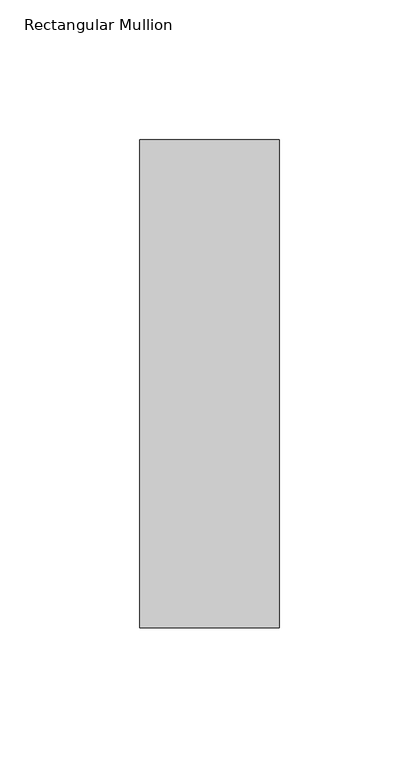
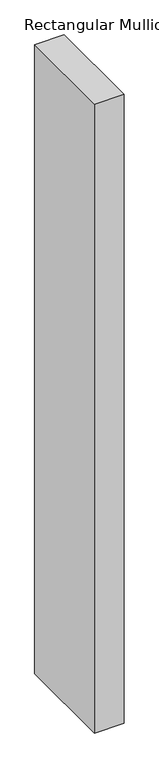
"""IFC4 building model written with IfcOpenShell, lengths in millimetres: member geometry, Rectangular Mullion : WWm-50x175-50mmOffset."""

from ifc_helpers import new_model, si_unit, frame, origin, place, context, project, spatial, polyline, outline, extrude, source, transform, mapped, element, save


def rectangular_mullion_8e94abb8(model_context):
    return source(origin(), model_context, "Body", "SweptSolid", [
        extrude(outline(polyline([(0.0, 87.5), (0.0, -87.5), (-50.0, -87.5), (-50.0, 87.5), (0.0, 87.5)])), frame((0.0, 0.0, -1125.0), z_axis=(0.0, 0.0, 1.0), x_axis=(1.0, 0.0, 0.0)), (0.0, 0.0, 1.0), 1125.0),
    ])


if __name__ == "__main__":
    model = new_model("IFC4")
    model_context = context("Model", 3, world=origin())
    ifc_project = project(units=[si_unit("LENGTHUNIT", "METRE", prefix="MILLI")], contexts=[model_context])
    site = spatial("IfcSite", under=ifc_project)
    building = spatial("IfcBuilding", under=site)
    placement = place(None, origin())
    rectangular_mullion_shape = rectangular_mullion_8e94abb8(model_context)
    element("IfcMember", 1, ObjectType="Rectangular Mullion : WWm-50x175-50mmOffset", at=placement, inside=building, context=model_context, shape_type="MappedRepresentation", body=[
        mapped(rectangular_mullion_shape, transform((0.0, 0.0, 0.0), x_axis=(1.0, 0.0, 0.0), y_axis=(0.0, 1.0, 0.0), z_axis=(0.0, 0.0, 1.0))),
    ])
    save(model, "model.ifc")

# Revit data of these elements
# Type "Rectangular Mullion : WWm-50x175-50mmOffset"
#   built-in parameter 1007304 = 0.574147 (stored number, unit not read)
#   built-in parameter 1007301 = 0.082021 (stored number, unit not read)
#   built-in parameter 1007300 = 0.082021 (stored number, unit not read)
# Element 1 (IfcMember, "Rectangular Mullion : WWm-50x175-50mmOffset")
#   Materials on its faces: "WW-EC-RGB-Mullion"
# Materials
#   "WW-EC-RGB-Mullion": class "Generic", colour RGB 255 255 255, transparency 0, Comments = "If region requests black mullions, switch asset color to RGB 25-25-25", Description = "Generic Color", Cost = 0
